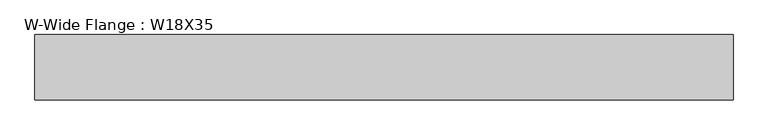
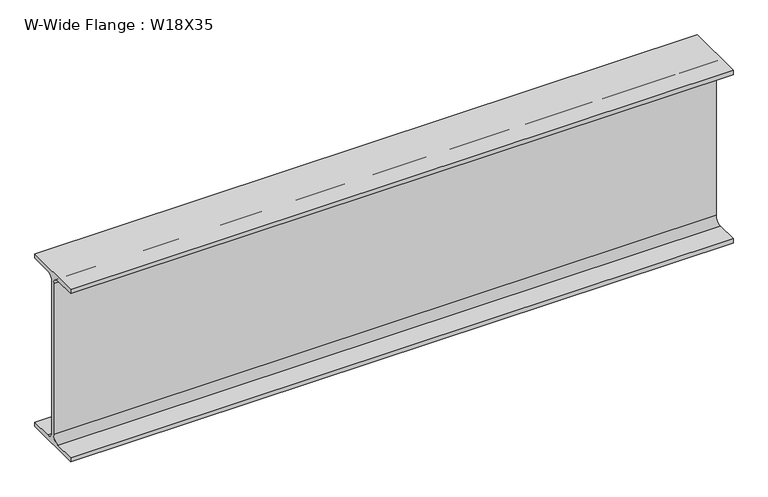
"""IFC4 building model written with IfcOpenShell, lengths in millimetres: beam geometry, W-Wide Flange : W18X35."""

from ifc_helpers import new_model, si_unit, point, frame, frame_2d, origin, place, context, project, spatial, polyline, circle_curve, trimmed, segment, composite_curve, outline, extrude, source, transform, mapped, element, save


def w_wide_flange_w18x35_3a39615e(model_context):
    return source(origin(), model_context, "Body", "SweptSolid", [
        extrude(outline(composite_curve([segment(polyline([(76.2, -213.995), (76.2, -224.79), (-76.2, -224.79), (-76.2, -213.995), (-21.59, -213.995)]), True, "CONTINUOUS"), segment(trimmed(circle_curve(frame_2d((-21.59, -196.215)), 17.78), [point((-21.59, -213.995))], [point((-3.81, -196.215))], True, "CARTESIAN"), True, "CONTINUOUS"), segment(polyline([(-3.81, -196.215), (-3.81, 196.215)]), True, "CONTINUOUS"), segment(trimmed(circle_curve(frame_2d((-21.59, 196.215)), 17.78), [point((-3.81, 196.215))], [point((-21.59, 213.995))], True, "CARTESIAN"), True, "CONTINUOUS"), segment(polyline([(-21.59, 213.995), (-76.2, 213.995), (-76.2, 224.79), (76.2, 224.79), (76.2, 213.995), (21.59, 213.995)]), True, "CONTINUOUS"), segment(trimmed(circle_curve(frame_2d((21.59, 196.215)), 17.78), [point((21.59, 213.995))], [point((3.81, 196.215))], True, "CARTESIAN"), True, "CONTINUOUS"), segment(polyline([(3.81, 196.215), (3.81, -196.215)]), True, "CONTINUOUS"), segment(trimmed(circle_curve(frame_2d((21.59, -196.215)), 17.78), [point((3.81, -196.215))], [point((21.59, -213.995))], True, "CARTESIAN"), True, "CONTINUOUS"), segment(polyline([(21.59, -213.995), (76.2, -213.995)]), True, "CONTINUOUS")], self_intersect=False)), frame((-825.5, 0.0, 0.0), z_axis=(1.0, 0.0, 0.0), x_axis=(0.0, 1.0, 0.0)), (0.0, 0.0, 1.0), 1631.95),
    ])


if __name__ == "__main__":
    model = new_model("IFC4")
    model_context = context("Model", 3, world=origin())
    ifc_project = project(units=[si_unit("LENGTHUNIT", "METRE", prefix="MILLI")], contexts=[model_context])
    site = spatial("IfcSite", under=ifc_project)
    building = spatial("IfcBuilding", under=site)
    placement = place(None, origin())
    w_wide_flange_w18x35_shape = w_wide_flange_w18x35_3a39615e(model_context)
    element("IfcBeam", 1, ObjectType="W-Wide Flange : W18X35", at=placement, inside=building, context=model_context, shape_type="MappedRepresentation", body=[
        mapped(w_wide_flange_w18x35_shape, transform((0.0, 0.0, 0.0), x_axis=(1.0, 0.0, 0.0), y_axis=(0.0, 1.0, 0.0), z_axis=(0.0, 0.0, 1.0))),
    ])
    save(model, "model.ifc")

# Revit data of these elements
# Type "W-Wide Flange : W18X35"
#   Assembly Code = "B10"
#   W = 35
#   Length [instance default] = 5' - 0"
#   bf = 0' - 6"
#   d = 1' - 5.7"
#   k = 0' - 1 1/8"
#   k2 = 0' - 0.7"
#   tf = 0' - 0.425"
#   tw = 0' - 0.3"
#   A = 0.0715278 SF
#   Structural Material [instance default] = Steel ASTM A992
# Element 1 (IfcBeam, "W-Wide Flange : W18X35")
#   Materials on its faces: "Steel ASTM A992"
# Materials
#   "Steel ASTM A992": class "Metal", colour RGB 199 199 199, transparency 0, Description = "Structural steel 50ksi", Cost = 0
